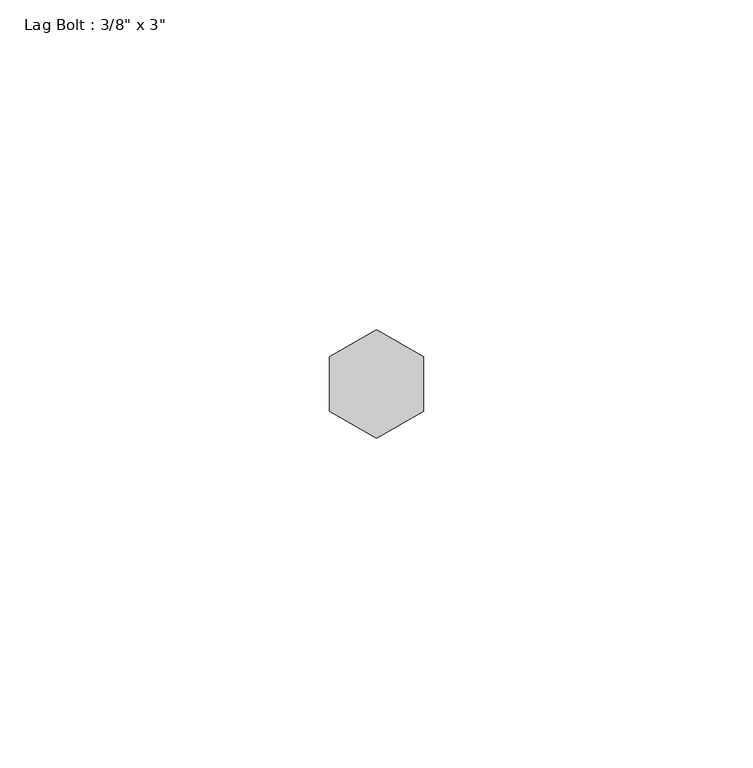
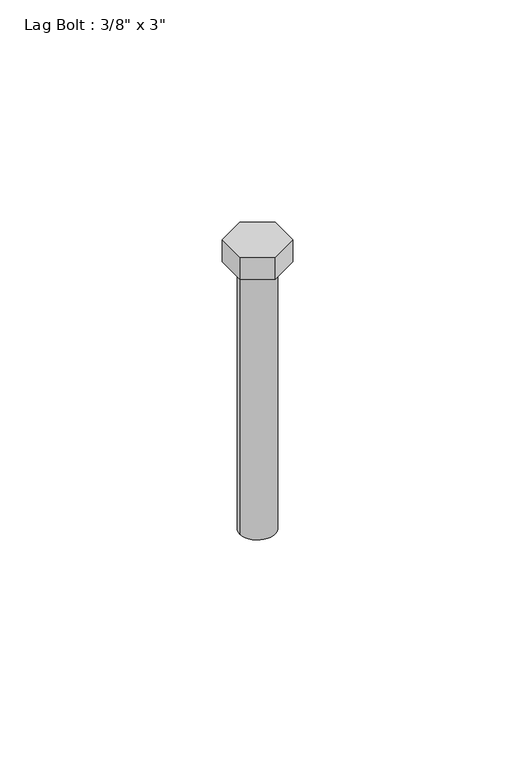
"""IFC4 building model written with IfcOpenShell, lengths in millimetres: proxy geometry."""

from ifc_helpers import new_model, si_unit, point, frame, origin, origin_with_axes, origin_2d, place, context, project, spatial, polyline, circle_curve, trimmed, segment, composite_curve, outline, extrude, source, transform, mapped, element, save


def proxy_8007053c(model_context):
    return source(origin(), model_context, "Body", "SweptSolid", [
        extrude(outline(polyline([(-7.14375, -4.124446), (-7.14375, 4.124446), (0.0, 8.248892), (7.14375, 4.124446), (7.14375, -4.124446), (0.0, -8.248892), (-7.14375, -4.124446)])), origin_with_axes(), (0.0, 0.0, 1.0), 6.35),
        extrude(outline(composite_curve([segment(trimmed(circle_curve(origin_2d(), 4.7625), [point((-4.7625, 0.0))], [point((4.7625, 0.0))], False, "CARTESIAN"), True, "CONTINUOUS"), segment(trimmed(circle_curve(origin_2d(), 4.7625), [point((4.7625, 0.0))], [point((-4.7625, 0.0))], False, "CARTESIAN"), True, "CONTINUOUS")], self_intersect=False)), frame((0.0, 0.0, -76.2), z_axis=(0.0, 0.0, 1.0), x_axis=(1.0, 0.0, 0.0)), (0.0, 0.0, 1.0), 76.2),
    ])


if __name__ == "__main__":
    model = new_model("IFC4")
    model_context = context("Model", 3, world=origin())
    ifc_project = project(units=[si_unit("LENGTHUNIT", "METRE", prefix="MILLI")], contexts=[model_context])
    site = spatial("IfcSite", under=ifc_project)
    building = spatial("IfcBuilding", under=site)
    placement = place(None, origin())
    proxy_shape = proxy_8007053c(model_context)
    element("IfcBuildingElementProxy", 1, Name="Lag Bolt : 3/8\" x 3\"", ObjectType="Lag Bolt : 3/8\" x 3\"", at=placement, inside=building, context=model_context, shape_type="MappedRepresentation", body=[
        mapped(proxy_shape, transform((0.0, 0.0, 0.0), x_axis=(1.0, 0.0, 0.0), y_axis=(0.0, 1.0, 0.0), z_axis=(0.0, 0.0, 1.0))),
    ])
    save(model, "model.ifc")

# Revit data of these elements
# Type "Lag Bolt : 3/8\" x 3\""
#   Thickness_of_Substrate [instance default] = 0' - 1"
#   Side = 0' - 0.3252"
#   Radius = 0' - 0 3/16"
#   Length = 0' - 3"
#   Head Size = 0' - 0 9/16"
#   Head Radius = 0' - 0 9/32"
#   Head Height = 0' - 0 1/4"
#   Diameter = 0' - 0 3/8"
#   Default Elevation = 4' - 0"
#   Nut_Visibility [instance default] = no
#   Bolt Material (Size) [instance default] = none
# Element 1 (IfcBuildingElementProxy, "Lag Bolt : 3/8\" x 3\"")
#   Bolt Material (Size) = _GALV. ANCHORS - SEE STRUCT. DWG
#   Materials on its faces: "_GALV. ANCHORS - SEE STRUCT. DWG"
# Materials
#   "_GALV. ANCHORS - SEE STRUCT. DWG": class "Generic", colour RGB 233 233 233, transparency 0, Cost = 0
